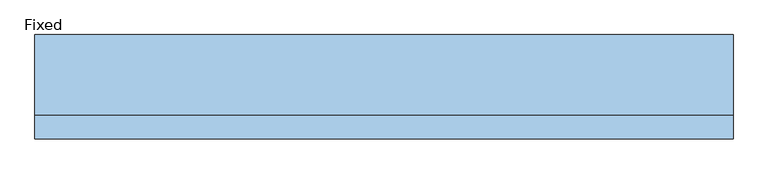
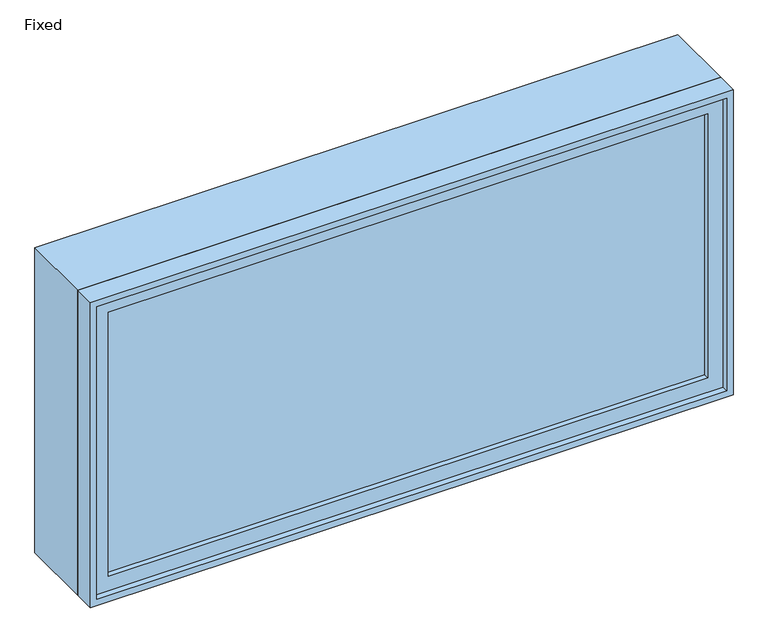
"""IFC4 building model written with IfcOpenShell, lengths in millimetres: window geometry, Fixed."""

import ifcopenshell
import ifcopenshell.guid

model = None  # the IFC model being written
_history = None  # IfcOwnerHistory: only IFC2X3 demands one
_inside = {}  # id of a spatial element -> (the spatial element, [elements in it])
_under = {}  # id of a project, library or spatial element -> (it, [spatial elements below it])
_declared = {}  # id of a project -> (the project, [libraries it declares])
_typed = {}  # id of a type object -> (the type object, [elements of that type])
_made_of = {}  # id of a material, layer set ... -> (it, [elements and type objects made of it])


def new_model(schema):
    """Start an empty IFC model of exactly this schema.

    Asked for "IFC4X3", IfcOpenShell would pick the latest addendum, in which some entities
    have other attributes; the version numbers below select the first issue.
    IFC2X3 requires an IfcOwnerHistory on every rooted entity: one is made here for all.
    """
    global model, _history
    if schema == "IFC4X3":
        model = ifcopenshell.file(schema_version=(4, 3, 0, 0))
    else:
        model = ifcopenshell.file(schema=schema)
    _inside.clear()
    _under.clear()
    _declared.clear()
    _typed.clear()
    _made_of.clear()
    _history = None
    if model.schema == "IFC2X3":
        org = make("IfcOrganization", Name="unknown")
        user = make(
            "IfcPersonAndOrganization",
            ThePerson=make("IfcPerson", FamilyName="unknown"),
            TheOrganization=org,
        )
        app = make(
            "IfcApplication",
            ApplicationDeveloper=org,
            Version="unknown",
            ApplicationFullName="unknown",
            ApplicationIdentifier="unknown",
        )
        _history = make(
            "IfcOwnerHistory",
            OwningUser=user,
            OwningApplication=app,
            ChangeAction="ADDED",
            CreationDate=0,
        )
    return model


def make(cls, **values):
    """One entity of the class cls with the attributes given. An attribute that is None is left unset."""
    return model.create_entity(
        cls, **{name: value for name, value in values.items() if value is not None}
    )


def rooted(cls, **values):
    """An entity with a GlobalId (a new one), such as an element, a storey or a relation."""
    return make(cls, GlobalId=ifcopenshell.guid.new(), OwnerHistory=_history, **values)


def si_unit(unit_type, name, prefix=None):
    """IfcSIUnit, for example si_unit("LENGTHUNIT", "METRE", prefix="MILLI")."""
    return make("IfcSIUnit", UnitType=unit_type, Prefix=prefix, Name=name)


def assignment(units):
    """IfcUnitAssignment: the units of a project."""
    return None if units is None else make("IfcUnitAssignment", Units=units)


def point(xyz):
    """IfcCartesianPoint."""
    return None if xyz is None else make("IfcCartesianPoint", Coordinates=xyz)


def direction(xyz):
    """IfcDirection."""
    return None if xyz is None else make("IfcDirection", DirectionRatios=xyz)


def frame(location, z_axis=None, x_axis=None):
    """IfcAxis2Placement3D, a coordinate frame: its origin and axes. An axis left out is left unset."""
    return make(
        "IfcAxis2Placement3D",
        Location=point(location),
        Axis=direction(z_axis),
        RefDirection=direction(x_axis),
    )


def origin():
    """The frame at (0, 0, 0) with its axes left unset."""
    return frame((0.0, 0.0, 0.0))


def place(relative_to, where):
    """IfcLocalPlacement: puts the frame where relative to a parent placement (None: the world)."""
    return make(
        "IfcLocalPlacement", PlacementRelTo=relative_to, RelativePlacement=where
    )


def context(
    kind, dimensions, precision=None, world=None, true_north=None, identifier=None
):
    """IfcGeometricRepresentationContext, for example the 3D "Model" context."""
    return make(
        "IfcGeometricRepresentationContext",
        ContextIdentifier=identifier,
        ContextType=kind,
        CoordinateSpaceDimension=dimensions,
        Precision=precision,
        WorldCoordinateSystem=world,
        TrueNorth=true_north,
    )


def project(units=None, contexts=None):
    """IfcProject with its units and contexts."""
    return rooted(
        "IfcProject",
        Name="project",
        RepresentationContexts=contexts,
        UnitsInContext=assignment(units),
    )


def spatial(cls, under=None, at=None, **own):
    """A site, building, storey or space (cls), placed at a placement, below another one or the project."""
    s = rooted(cls, ObjectPlacement=at, **own)
    if under is not None:
        _under.setdefault(under.id(), (under, []))[1].append(s)
    return s


def polyline(points):
    """IfcPolyline through the points."""
    return make("IfcPolyline", Points=[point(p) for p in points])


def outline(outer, holes=None, kind="AREA"):
    """IfcArbitraryClosedProfileDef: a profile drawn as a closed curve; with holes, ...WithVoids."""
    if holes is None:
        return make("IfcArbitraryClosedProfileDef", ProfileType=kind, OuterCurve=outer)
    return make(
        "IfcArbitraryProfileDefWithVoids",
        ProfileType=kind,
        OuterCurve=outer,
        InnerCurves=holes,
    )


def extrude(swept, where, along, depth):
    """IfcExtrudedAreaSolid: the profile swept, set in the frame where, extruded along a direction by depth."""
    return make(
        "IfcExtrudedAreaSolid",
        SweptArea=swept,
        Position=where,
        ExtrudedDirection=direction(along),
        Depth=depth,
    )


def shape(context_of_items, identifier, shape_type, items):
    """IfcShapeRepresentation: the items that make up one representation, for example the "Body"."""
    return make(
        "IfcShapeRepresentation",
        ContextOfItems=context_of_items,
        RepresentationIdentifier=identifier,
        RepresentationType=shape_type,
        Items=items,
    )


def source(mapping_origin, context_of_items, identifier, shape_type, items):
    """IfcRepresentationMap: a shape defined once, which mapped items show again and again."""
    return make(
        "IfcRepresentationMap",
        MappingOrigin=mapping_origin,
        MappedRepresentation=shape(context_of_items, identifier, shape_type, items),
    )


def transform(
    local_origin,
    x_axis=None,
    y_axis=None,
    z_axis=None,
    scale=None,
    scale2=None,
    scale3=None,
    uniform=True,
):
    """IfcCartesianTransformationOperator3D, or its non-uniform kind. x_axis, y_axis, z_axis: its Axis1, 2, 3."""
    if uniform:
        return make(
            "IfcCartesianTransformationOperator3D",
            Axis1=direction(x_axis),
            Axis2=direction(y_axis),
            LocalOrigin=point(local_origin),
            Scale=scale,
            Axis3=direction(z_axis),
        )
    return make(
        "IfcCartesianTransformationOperator3DnonUniform",
        Axis1=direction(x_axis),
        Axis2=direction(y_axis),
        LocalOrigin=point(local_origin),
        Scale=scale,
        Axis3=direction(z_axis),
        Scale2=scale2,
        Scale3=scale3,
    )


def mapped(mapping_source, mapping_target):
    """IfcMappedItem: shows the shape of a source again, moved by a transform."""
    return make(
        "IfcMappedItem", MappingSource=mapping_source, MappingTarget=mapping_target
    )


def made_of(thing, what):
    """Note that an element or type object is made of a material, layer set ...; save() writes the relation."""
    if what is not None:
        _made_of.setdefault(what.id(), (what, []))[1].append(thing)
    return thing


def element(
    cls,
    number,
    at=None,
    inside=None,
    cuts=None,
    type_object=None,
    material=None,
    context=None,
    identifier="Body",
    shape_type=None,
    held_by="IfcProductDefinitionShape",
    body=None,
    shapes=None,
    **own,
):
    """One element of the class cls, such as IfcWall. Its Tag is "e" and its number.

    at: its placement. inside: the storey or other place that contains it. cuts: it is an
    opening in that element (IfcRelVoidsElement). A single representation is given by context,
    identifier, shape_type and body (its items); several are given by shapes. held_by: the class
    of the entity that holds the representations. save() writes the other relations.
    """
    e = rooted(cls, Tag="e%d" % number, ObjectPlacement=at, **own)
    if body is not None:
        shapes = [shape(context, identifier, shape_type, body)]
    if shapes is not None:
        e.Representation = make(held_by, Representations=shapes)
    if inside is not None:
        _inside.setdefault(inside.id(), (inside, []))[1].append(e)
    if cuts is not None:
        rooted(
            "IfcRelVoidsElement", RelatingBuildingElement=cuts, RelatedOpeningElement=e
        )
    if type_object is not None:
        _typed.setdefault(type_object.id(), (type_object, []))[1].append(e)
    return made_of(e, material)


def aggregate(whole, parts):
    """IfcRelAggregates: a whole, such as a stair, and the parts it consists of."""
    return rooted("IfcRelAggregates", RelatingObject=whole, RelatedObjects=parts)


def save(model, path):
    """Write the relations noted so far, then the file.

    IfcRelAggregates (storeys below a building ...), IfcRelContainedInSpatialStructure (elements
    in a storey), IfcRelDefinesByType, IfcRelAssociatesMaterial and IfcRelDeclares: one each for
    every whole, place, type object, material and project.
    """
    for whole, parts in _under.values():
        aggregate(whole, parts)
    for where, things in _inside.values():
        rooted(
            "IfcRelContainedInSpatialStructure",
            RelatedElements=things,
            RelatingStructure=where,
        )
    for kind, things in _typed.values():
        rooted("IfcRelDefinesByType", RelatedObjects=things, RelatingType=kind)
    for what, things in _made_of.values():
        rooted("IfcRelAssociatesMaterial", RelatedObjects=things, RelatingMaterial=what)
    for by, libraries in _declared.values():
        rooted("IfcRelDeclares", RelatingContext=by, RelatedDefinitions=libraries)
    model.write(path)


def fixed_06ce57b0(model_context):
    return source(origin(), model_context, "Body", "SweptSolid", [
        extrude(outline(polyline([(835.025, -92.075), (835.025, -104.775), (-911.225, -104.775), (-911.225, -92.075), (835.025, -92.075)])), frame((0.0, 0.0, 1257.3), z_axis=(0.0, 0.0, 1.0), x_axis=(1.0, 0.0, 0.0)), (0.0, 0.0, 1.0), 812.8),
        extrude(outline(polyline([(2114.55, -955.675), (1212.85, -955.675), (1212.85, 879.475), (2114.55, 879.475), (2114.55, -955.675)]), holes=[polyline([(2070.1, -911.225), (2070.1, 835.025), (1257.3, 835.025), (1257.3, -911.225), (2070.1, -911.225)])]), frame((0.0, -120.65, 0.0), z_axis=(0.0, 1.0, 0.0), x_axis=(0.0, 0.0, 1.0)), (0.0, 0.0, 1.0), 44.45),
        extrude(outline(polyline([(2133.6, -974.725), (1193.8, -974.725), (1193.8, 898.525), (2133.6, 898.525), (2133.6, -974.725)]), holes=[polyline([(2101.85, -942.975), (2101.85, 866.775), (1225.55, 866.775), (1225.55, -942.975), (2101.85, -942.975)])]), frame((0.0, -76.2, 0.0), z_axis=(0.0, 1.0, 0.0), x_axis=(0.0, 0.0, 1.0)), (0.0, 0.0, 1.0), 215.9),
        extrude(outline(polyline([(2133.6, 898.525), (2133.6, -974.725), (1193.8, -974.725), (1193.8, 898.525), (2133.6, 898.525)]), holes=[polyline([(2114.55, 879.475), (1212.85, 879.475), (1212.85, -955.675), (2114.55, -955.675), (2114.55, 879.475)])]), frame((0.0, -139.7, 0.0), z_axis=(0.0, 1.0, 0.0), x_axis=(0.0, 0.0, 1.0)), (0.0, 0.0, 1.0), 63.5),
    ])


if __name__ == "__main__":
    model = new_model("IFC4")
    model_context = context("Model", 3, world=origin())
    ifc_project = project(units=[si_unit("LENGTHUNIT", "METRE", prefix="MILLI")], contexts=[model_context])
    site = spatial("IfcSite", under=ifc_project)
    building = spatial("IfcBuilding", under=site)
    placement = place(None, origin())
    fixed_shape = fixed_06ce57b0(model_context)
    element("IfcWindow", 1, ObjectType="Fixed : 6' 1 34\"\" x 3' 1\"", at=placement, inside=building, context=model_context, shape_type="MappedRepresentation", body=[
        mapped(fixed_shape, transform((0.0, 0.0, 0.0), x_axis=(1.0, 0.0, 0.0), y_axis=(0.0, 1.0, 0.0), z_axis=(0.0, 0.0, 1.0))),
    ])
    save(model, "model.ifc")

# Revit data of these elements
# Type "Fixed : 6' 1 34\"\" x 3' 1\""
#   Type Mark = "10"
#   Assembly Code = "B2020100"
#   Height = 3' - 1"
#   Default Sill Height = 3' - 11"
#   Width = 6' - 1 3/4"
#   Window Inset = 0' - 0 3/4"
#   Glass Pane Material = Glass
#   Sash Material = accent 2
#   Wall Closure = (empty or 0)
# Element 1 (IfcWindow, "Fixed : 6' 1 34\"\" x 3' 1\"")
#   Materials on its faces: "accent 2", "Glass"
# Materials
#   "Glass": class "Glass", colour RGB 236 240 239, transparency 0.85, Description = "Soda Lime Glass", Cost = 0
#   "accent 2": class "Wood", colour RGB 80 80 80, transparency 0, Description = "Wood framing, thermal airspace", Cost = 0
